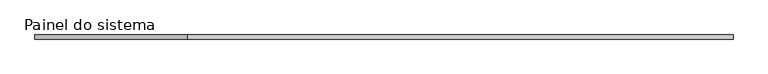
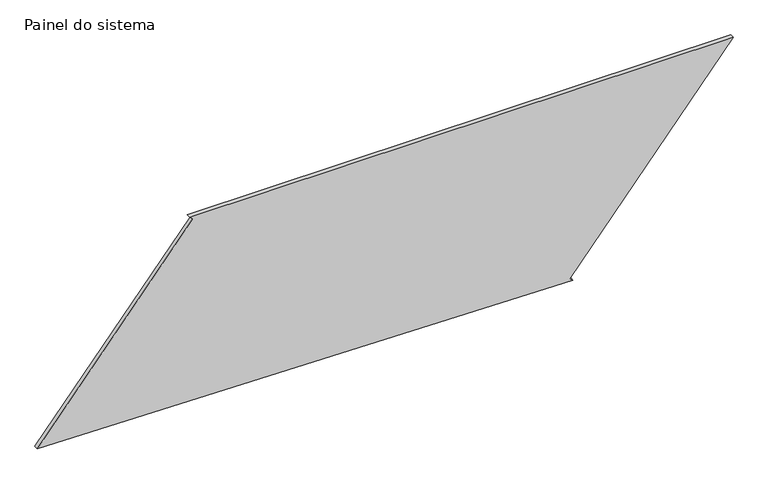
"""IFC4 building model written with IfcOpenShell, lengths in millimetres: plate geometry, Painel do sistema : Envidraçado."""

from ifc_helpers import new_model, si_unit, frame, origin, place, context, project, spatial, polyline, outline, extrude, source, transform, mapped, element, save


def painel_do_sistema_eb259335(model_context):
    return source(origin(), model_context, "Body", "SweptSolid", [
        extrude(outline(polyline([(0.0, 1140.8028868), (15.8992441, 1121.5100374), (1219.79577, 2113.6415968), (1219.79577, -1187.6190003), (1203.8965259, -1168.326151), (56.8087527, -2113.6415968), (0.0, 1140.8028868)])), frame((0.0, 24.5, 0.0), z_axis=(0.0, 1.0, 0.0), x_axis=(0.0, 0.0, 1.0)), (0.0, 0.0, 1.0), 25.0),
    ])


if __name__ == "__main__":
    model = new_model("IFC4")
    model_context = context("Model", 3, world=origin())
    ifc_project = project(units=[si_unit("LENGTHUNIT", "METRE", prefix="MILLI")], contexts=[model_context])
    site = spatial("IfcSite", under=ifc_project)
    building = spatial("IfcBuilding", under=site)
    placement = place(None, origin())
    painel_do_sistema_shape = painel_do_sistema_eb259335(model_context)
    element("IfcPlate", 1, ObjectType="Painel do sistema : Envidraçado", at=placement, inside=building, context=model_context, shape_type="MappedRepresentation", body=[
        mapped(painel_do_sistema_shape, transform((0.0, 0.0, 0.0), x_axis=(1.0, 0.0, 0.0), y_axis=(0.0, 1.0, 0.0), z_axis=(0.0, 0.0, 1.0))),
    ])
    save(model, "model.ifc")

# Revit data of these elements
# Type "Painel do sistema : Envidraçado"
#   Construction Type Id = "GSP4R"
#   Analytic Construction = "Vidraça única Pilkington 1/8 pol"
#   Visual Light Transmittance = 0.9
#   Solar Heat Gain Coefficient = 0.86
#   Heat Transfer Coefficient (U) = 6.7069 W/(m²·K)
# Element 1 (IfcPlate, "Painel do sistema : Envidraçado")
#   Materials on its faces: "Vidro"
# Materials
#   "Vidro": class "Vidro", colour RGB 0 128 192, transparency 0.9, Description = "Vidro de sílica", Cost = 0
